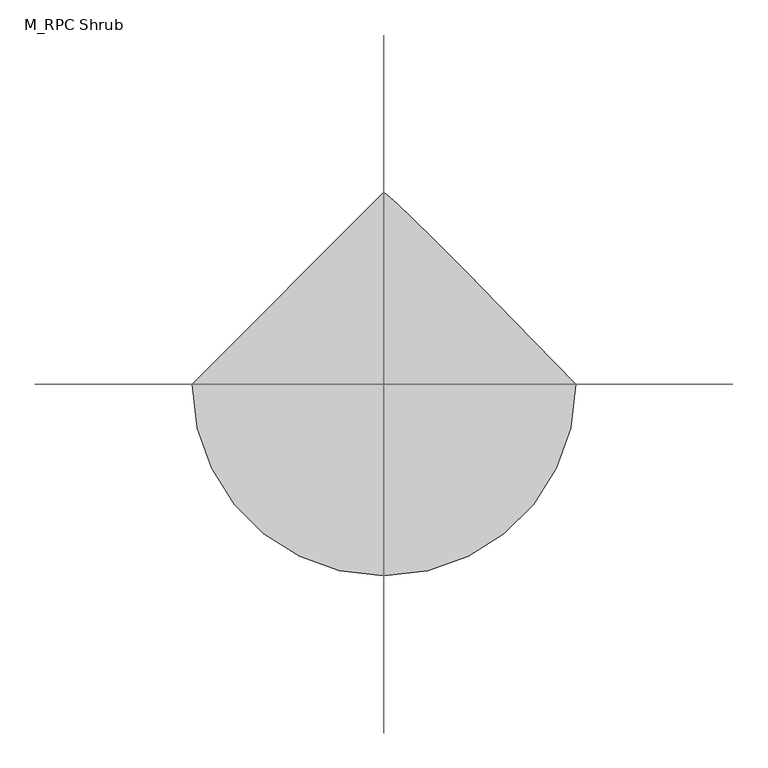
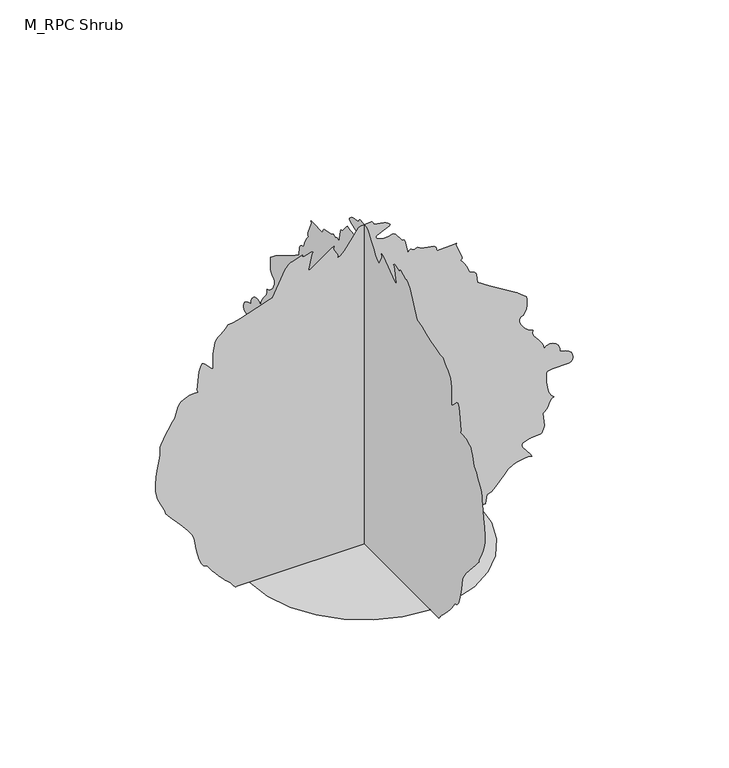
"""IFC4 building model written with IfcOpenShell, lengths in millimetres: geographic element geometry, M_RPC Shrub : Vibernum - 0.92 Meters."""

from ifc_helpers import new_model, si_unit, origin, place, context, project, spatial, triangles, source, transform, mapped, element, save


def m_rpc_shrub_8dd75232(model_context):
    return source(origin(), model_context, "Body", "Tessellation", [
        triangles([(-312.3019403, 0.0, 0.0), (-304.047466, -71.5591904, 0.0), (-280.533785, -137.2748422, 0.0), (-243.6445759, -195.2642804, 0.0), (-195.2642804, -243.6445759, 0.0), (-137.2748422, -280.533785, 0.0), (-71.5591904, -304.047466, 0.0), (1.37e-05, -312.3019403, 0.0), (71.5591904, -304.047466, 0.0), (137.2748422, -280.533785, 0.0), (195.2642804, -243.6445759, 0.0), (243.6445759, -195.2642804, 0.0), (280.533785, -137.2748422, 0.0), (304.047466, -71.5591904, 0.0), (312.3019403, 2.73e-05, 0.0), (210.8115327, 104.1055005, 0.0), (135.5708038, 180.7538289, 0.0), (82.2056472, 234.5209685, 0.0), (46.341203, 269.9844471, 0.0), (23.602184, 291.7169141, 0.0), (9.6134973, 304.2979231, 0.0), (-4.1e-05, 312.3019403, 0.0), (-354.9158363, 2.17e-05, 4.3761881), (-358.1767565, 2.14e-05, 8.534566), (-361.2817268, 2.12e-05, 12.3988753), (-364.2359797, 2.1e-05, 15.8927061), (-367.0419857, 2.08e-05, 18.9398516), (-369.7074117, 2.06e-05, 21.4638743), (-372.2322939, 2.05e-05, 23.3884638), (-378.1177631, 2.02e-05, 28.7068347), (-385.9096567, 1.97e-05, 36.5531626), (-394.8617629, 1.91e-05, 46.1891501), (-404.2381165, 1.85e-05, 56.876234), (-413.2898895, 1.79e-05, 67.8763802), (-421.2734502, 1.73e-05, 78.4512797), (-427.4502534, 1.67e-05, 87.8626239), (-436.9799043, 1.65e-05, 90.8633673), (-444.2223764, 1.6e-05, 99.7947807), (-449.6503881, 1.52e-05, 113.1020808), (-453.7290273, 1.42e-05, 129.2314832), (-456.9337008, 1.32e-05, 146.6279323), (-459.7294968, 1.22e-05, 163.737135), (-462.5891696, 1.12e-05, 179.0048078), (-468.7352697, 1.05e-05, 190.9709378), (-479.8672937, 9.6e-06, 206.3408391), (-493.9688676, 8.6e-06, 223.4354715), (-509.0261971, 7.6e-06, 240.5755953), (-523.0229808, 6.6e-06, 256.082207), (-533.9428811, 5.9e-06, 268.2773383), (-539.7695603, 5.5e-06, 275.4814407), (-541.2747737, 5.1e-06, 281.6198924), (-544.5919041, 4.7e-06, 289.5319094), (-548.9951237, 4.1e-06, 298.5044722), (-553.7612208, 3.6e-06, 307.832264), (-558.1644768, 3e-06, 316.8048268), (-561.4815708, 2.6e-06, 324.7142641), (-562.9867842, 2.2e-06, 330.8552773), (-567.5177939, 1.1e-06, 348.3710687), (-568.1004619, -1e-07, 369.3445341), (-565.9844573, -1.4e-06, 391.9765466), (-562.4143627, -2.8e-06, 414.4603486), (-558.6398111, -4e-06, 434.9916899), (-555.9053487, -5e-06, 451.7663564), (-555.4581376, -5.7e-06, 462.9801704), (-554.8294696, -6.3e-06, 472.6580681), (-551.5404625, -6.9e-06, 482.7883), (-546.3679948, -7.5e-06, 493.1791992), (-540.0966843, -8.1e-06, 503.6441854), (-533.5084236, -8.7e-06, 513.9839613), (-527.387867, -9.3e-06, 524.0119829), (-522.5144362, -9.9e-06, 533.5340034), (-517.8479696, -1.01e-05, 537.8503461), (-514.3085418, -1.06e-05, 545.0212383), (-511.4412023, -1.11e-05, 553.9068878), (-508.8013198, -1.17e-05, 563.3599082), (-505.9365237, -1.22e-05, 572.2430142), (-502.3945161, -1.26e-05, 579.4139065), (-497.7280858, -1.29e-05, 583.7328289), (-491.707196, -1.31e-05, 586.9451328), (-486.0159737, -1.33e-05, 589.7204721), (-480.370715, -1.34e-05, 591.9949336), (-474.4878256, -1.35e-05, 593.6994807), (-468.0810582, -1.35e-05, 594.7651497), (-460.8615861, -1.35e-05, 595.1254838), (-452.5509378, -1.35e-05, 594.7140627), (-454.8586095, -1.39e-05, 601.4453742), (-449.5864749, -1.7e-05, 652.1016209), (-445.5359227, -1.76e-05, 663.7626823), (-440.7468255, -1.81e-05, 672.2471209), (-437.1766946, -1.81e-05, 671.6951197), (-433.6142303, -1.8e-05, 669.1088676), (-417.0644411, -1.69e-05, 651.3937426), (-411.7642196, -1.67e-05, 648.3628956), (-411.5010089, -1.75e-05, 661.4268511), (-411.6236758, -1.81e-05, 670.3457834), (-411.8281328, -1.84e-05, 676.8215509), (-411.8102197, -1.88e-05, 682.5587734), (-411.2658852, -1.92e-05, 689.2594545), (-409.888462, -1.97e-05, 698.6281414), (-407.3712101, -2.05e-05, 712.3668377), (-405.7612066, -2.11e-05, 721.8709087), (-402.254989, -2.15e-05, 728.7811701), (-397.2435579, -2.18e-05, 734.1146381), (-391.1102114, -2.21e-05, 738.888402), (-384.2485299, -2.24e-05, 744.1247103), (-377.041884, -2.28e-05, 750.8407248), (-369.8786222, -2.34e-05, 760.056078), (-356.6894199, -2.34e-05, 760.8763767), (-337.3923783, -2.37e-05, 765.7038437), (-314.8319095, -2.42e-05, 772.9769463), (-291.8651246, -2.47e-05, 781.1368406), (-271.3388884, -2.51e-05, 788.6195234), (-256.1026636, -2.54e-05, 793.8635347), (-249.0097099, -2.55e-05, 795.3125742), (-214.9880765, -2.96e-05, 864.0289467), (-206.5153742, -3.02e-05, 874.8747236), (-198.5757789, -3.05e-05, 879.4338203), (-194.4166032, -3.05e-05, 879.2012764), (-169.7628755, -3.11e-05, 889.5334219), (-167.4802568, -3.11e-05, 888.8663841), (-169.1035589, -3.08e-05, 884.473411), (-162.8687651, -3.08e-05, 884.7749187), (-145.2576398, -3.11e-05, 890.2566336), (-141.9579048, -3.11e-05, 889.5691755), (-138.8076701, -3.09e-05, 886.8066261), (-141.6543078, -3.09e-05, 885.8252907), (-151.2105559, -2.84e-05, 843.1832714), (-151.3572493, -2.81e-05, 839.1173859), (-142.906784, -2.83e-05, 842.4907265), (-90.4708313, -3.06e-05, 880.7678232), (-82.020366, -3.08e-05, 884.1411638), (-83.7461328, -3.04e-05, 878.3323614), (-82.5360776, -3.01e-05, 872.9759296), (-73.0337507, -2.92e-05, 857.8138464), (-71.8234367, -2.89e-05, 852.457342), (-73.5492034, -2.85e-05, 846.6486122), (-63.9454201, -2.88e-05, 850.7834616), (-53.4106434, -2.94e-05, 861.4529411), (-42.6269584, -3.03e-05, 875.9301825), (-32.2761822, -3.12e-05, 891.4755999), (-23.0409855, -3.21e-05, 905.3650864), (-15.602804, -3.26e-05, 914.8640705), (-10.6438464, -3.27e-05, 917.2407423), (19.0264334, -3.29e-05, 920.0007483), (21.6640755, -3.29e-05, 918.7715355), (24.0025888, -3.27e-05, 915.4569849), (26.8484339, -3.23e-05, 909.3977617), (53.6932888, -3.21e-05, 905.3395065), (59.1330503, -3.19e-05, 902.9602913), (64.3586534, -3.17e-05, 899.3978634), (69.5170458, -3.14e-05, 894.3378525), (68.476934, -3.12e-05, 890.9466351), (63.7141433, -3.1e-05, 887.5732944), (34.9342185, -3.03e-05, 875.4190218), (32.1818815, -3.01e-05, 873.0040529), (32.3303599, -2.99e-05, 869.0122908), (35.7864966, -2.97e-05, 865.4217396), (41.7820881, -2.95e-05, 862.5365232), (49.5489423, -2.94e-05, 860.6632364), (58.3180791, -2.94e-05, 860.1163948), (67.3220762, -2.94e-05, 861.1973608), (75.7922169, -2.96e-05, 864.218034), (80.0229407, -2.96e-05, 864.2512442), (84.706512, -2.94e-05, 860.3745186), (99.6636841, -2.82e-05, 840.924107), (104.3475097, -2.8e-05, 837.0473814), (108.5782381, -2.8e-05, 837.0780481), (111.2337173, -2.77e-05, 832.0333706), (118.4610832, -2.55e-05, 796.4497868), (122.8172944, -2.58e-05, 801.0931807), (126.0518626, -2.59e-05, 802.5371332), (128.7277803, -2.59e-05, 801.9544653), (134.6612753, -2.58e-05, 799.3784597), (139.0463547, -2.58e-05, 799.7259676), (145.1290957, -2.59e-05, 802.7236771), (155.0420989, -2.55e-05, 796.4983303), (189.6435843, -2.52e-05, 789.5906851), (194.7493409, -2.48e-05, 784.3466738), (197.5241715, -2.42e-05, 774.4873192), (244.8328936, -2.43e-05, 775.7599886), (250.8604327, -2.44e-05, 776.9968317), (249.2693416, -2.41e-05, 771.5561028), (265.3001036, -2.18e-05, 733.5293541), (266.0080001, -2.14e-05, 726.8210426), (261.8424295, -2.12e-05, 723.9741234), (266.0591053, -2.1e-05, 720.0232744), (270.234886, -2.07e-05, 714.4291391), (274.257333, -2.03e-05, 707.7387045), (278.0191129, -1.98e-05, 700.503899), (281.4077868, -1.94e-05, 693.2690935), (284.3134598, -1.9e-05, 686.5812023), (286.6262365, -1.87e-05, 680.9922266), (293.9427957, -1.85e-05, 678.6513084), (299.3426841, -1.83e-05, 675.7763386), (303.1223589, -1.81e-05, 672.1142075), (305.5782592, -1.79e-05, 667.414567), (307.9625977, -1.65e-05, 644.5985178), (339.6157165, -1.52e-05, 623.0781744), (415.3650172, -1.24e-05, 576.2961462), (440.8030357, -1.13e-05, 556.8688073), (442.576583, -1.09e-05, 550.3086699), (442.6839166, -9.8e-06, 531.5483325), (440.8055792, -9.2e-06, 521.6711011), (437.4961518, -8.7e-06, 513.0077491), (432.650808, -8.3e-06, 506.7185254), (426.1647941, -8.1e-06, 503.9636427), (422.1781188, -7.8e-06, 498.3005073), (422.533366, -7.3e-06, 490.1891928), (426.3513379, -6.7e-06, 480.8102958), (432.7453517, -6.2e-06, 471.3393986), (440.8337025, -5.7e-06, 462.9545906), (449.7321419, -5.3e-06, 456.834034), (458.5564942, -5.1e-06, 454.1558181), (457.3502815, -4.7e-06, 446.192714), (460.7465858, -4.2e-06, 437.8002394), (467.069056, -3.7e-06, 429.0065901), (474.6386158, -3.1e-06, 419.8346935), (481.7788413, -2.5e-06, 410.312673), (486.8081855, -1.9e-06, 400.4635649), (488.0501882, -1.3e-06, 390.3103329), (495.6350813, -1.7e-06, 396.7784337), (504.4108538, -1.9e-06, 398.9378949), (513.4166631, -1.8e-06, 397.4173119), (521.6864345, -1.5e-06, 392.8454252), (528.2618689, -1.1e-06, 385.8534465), (532.179544, -5e-07, 377.0725508), (532.4734214, 0.0, 367.1314061), (546.6107852, 2e-07, 363.8347323), (556.6388068, 5e-07, 359.145302), (563.158031, 8e-07, 353.5384131), (566.7767055, 1.2e-06, 347.4894001), (568.1004619, 1.6e-06, 341.476177), (567.7299176, 1.9e-06, 335.9714985), (566.2732478, 2.1e-06, 331.4558221), (561.9262384, 2.4e-06, 327.0142691), (555.0594701, 2.5e-06, 325.3173886), (511.4182022, 2.5e-06, 325.4477222), (498.7170879, 2.7e-06, 322.0718382), (496.0746257, 3e-06, 317.2162479), (494.9374131, 3.7e-06, 306.5493482), (495.402501, 4.5e-06, 292.2791255), (497.5721724, 5.4e-06, 276.6186715), (501.5384274, 6.3e-06, 261.7785526), (507.4034037, 7e-06, 249.9677909), (515.2668772, 7.4e-06, 243.4002594), (509.294531, 7.7e-06, 239.3864964), (505.0855219, 8e-06, 233.7990286), (501.9447616, 8.4e-06, 227.2979356), (499.1745091, 8.8e-06, 220.5436059), (496.0848358, 9.1e-06, 214.1955922), (491.9806169, 9.5e-06, 208.9140286), (486.1667275, 9.7e-06, 205.3589949), (489.4889448, 1.19e-05, 168.9520057), (487.7639411, 1.24e-05, 160.1419693), (482.6553866, 1.3e-05, 150.3409051), (480.9687163, 1.31e-05, 148.301313), (450.9639344, 1.32e-05, 146.2540543), (429.6940118, 1.36e-05, 139.4731364), (428.2807986, 1.4e-05, 133.6410978), (430.2076796, 1.43e-05, 127.5542691), (451.9478133, 1.59e-05, 100.1517902), (456.0469454, 1.64e-05, 92.4117739), (449.7219317, 1.63e-05, 94.6872437), (435.3801473, 1.63e-05, 94.8479897), (418.8610248, 1.65e-05, 90.6992967), (417.1436877, 1.66e-05, 89.9019616), (403.775572, 1.67e-05, 86.4391824), (391.3376684, 1.73e-05, 77.4489881), (379.5693097, 1.81e-05, 65.0972075), (368.2072852, 1.89e-05, 51.5494334), (356.9832973, 1.96e-05, 38.9722533), (345.6366062, 2.02e-05, 29.5310031), (333.9040375, 2.04e-05, 25.3916891), (328.9564834, 2.19e-05, 4.03e-05), (-351.4939522, 2.19e-05, 4.03e-05), (-4.6e-06, -354.9158363, 4.3762136), (-4.6e-06, -358.1767565, 8.5345916), (-4.6e-06, -361.2817268, 12.3988753), (-4.6e-06, -364.2359797, 15.8927322), (-4.6e-06, -367.0419857, 18.9398766), (-4.6e-06, -369.7074117, 21.4638993), (-4.6e-06, -372.2322939, 23.3884638), (-4.6e-06, -378.1177631, 28.7068347), (-4.6e-06, -385.9096567, 36.5531626), (-4.6e-06, -394.8617629, 46.1891501), (-4.6e-06, -404.2381165, 56.876234), (-4.6e-06, -413.2898895, 67.8766345), (-4.6e-06, -421.2734502, 78.4512797), (-4.6e-06, -427.4502534, 87.8626239), (-4.6e-06, -436.9799043, 90.8633673), (-4.6e-06, -444.2223764, 99.7947807), (-4.6e-06, -449.6503881, 113.1023351), (-4.6e-06, -453.7290273, 129.2314832), (-4.6e-06, -456.9337008, 146.6279323), (-4.6e-06, -459.7294968, 163.737135), (-4.6e-06, -462.5891696, 179.0048078), (-4.6e-06, -468.7352697, 190.9709378), (-4.6e-06, -479.8672937, 206.3408391), (-4.6e-06, -493.9688676, 223.4354715), (-4.6e-06, -509.0261971, 240.5755953), (-4.6e-06, -523.0229808, 256.082207), (-4.6e-06, -533.9428811, 268.2773383), (-4.6e-06, -539.7695603, 275.4814407), (-4.6e-06, -541.2747737, 281.6198924), (-4.6e-06, -544.5919041, 289.5319094), (-4.6e-06, -548.9951237, 298.5044722), (-4.6e-06, -553.7612208, 307.832264), (-4.6e-06, -558.1644768, 316.8048268), (-4.6e-06, -561.4815708, 324.7142641), (-4.6e-06, -562.9867842, 330.8552773), (-4.6e-06, -567.5177939, 348.3710687), (-4.6e-06, -568.1004619, 369.3445341), (-4.6e-06, -565.9844573, 391.9765466), (-4.6e-06, -562.4143627, 414.4603486), (-4.6e-06, -558.6398111, 434.9916899), (-4.6e-06, -555.9053487, 451.7663564), (-4.6e-06, -555.4581376, 462.9801704), (-4.6e-06, -554.8294696, 472.6580681), (-4.6e-06, -551.5404625, 482.7883), (-4.6e-06, -546.3679948, 493.1791992), (-4.6e-06, -540.0966843, 503.6441854), (-4.6e-06, -533.5084236, 513.9839613), (-4.6e-06, -527.387867, 524.0119829), (-4.6e-06, -522.5144362, 533.5340034), (-4.6e-06, -517.8479696, 537.8503461), (-4.6e-06, -514.3085418, 545.0212383), (-4.6e-06, -511.4412023, 553.9068878), (-4.6e-06, -508.8013198, 563.3599082), (-4.6e-06, -505.9365237, 572.2430142), (-4.6e-06, -502.3945161, 579.4164863), (-4.6e-06, -497.7280858, 583.7328289), (-4.6e-06, -491.707196, 586.9451328), (-4.6e-06, -486.0159737, 589.7204721), (-4.6e-06, -480.370715, 591.9949336), (-4.6e-06, -474.4878256, 593.6994807), (-4.6e-06, -468.0810582, 594.7651497), (-4.6e-06, -460.8615861, 595.1254838), (-4.6e-06, -452.5509378, 594.7140627), (-4.6e-06, -454.8586095, 601.4453742), (-4.6e-06, -449.5864749, 652.1016209), (-4.6e-06, -445.5359227, 663.7626823), (-4.6e-06, -440.7468255, 672.2471209), (-4.6e-06, -437.1766946, 671.6951197), (-4.6e-06, -433.6142303, 669.1088676), (-4.6e-06, -417.0644411, 651.3937426), (-4.6e-06, -411.7642196, 648.3628956), (-4.6e-06, -411.5010089, 661.4268511), (-4.6e-06, -411.6236758, 670.3457834), (-4.6e-06, -411.8281328, 676.8215509), (-4.6e-06, -411.8102197, 682.5587734), (-4.6e-06, -411.2658852, 689.2594545), (-4.6e-06, -409.888462, 698.6281414), (-4.6e-06, -407.3712101, 712.3668377), (-4.6e-06, -405.7612066, 721.8709087), (-4.6e-06, -402.254989, 728.7811701), (-4.6e-06, -397.2435579, 734.1146381), (-4.6e-06, -391.1102114, 738.888402), (-4.6e-06, -384.2485299, 744.1247103), (-4.6e-06, -377.041884, 750.8407248), (-4.6e-06, -369.8786222, 760.056078), (-4.6e-06, -356.6894199, 760.8763767), (-4.6e-06, -337.3923783, 765.7038437), (-4.6e-06, -314.8319095, 772.9769463), (-4.6e-06, -291.8651246, 781.1368406), (-4.6e-06, -271.3388884, 788.6195234), (-4.6e-06, -256.1026636, 793.8635347), (-4.6e-06, -249.0097099, 795.3125742), (-4.6e-06, -214.9880765, 864.0289467), (-4.6e-06, -206.5153742, 874.8747236), (-4.6e-06, -198.5757789, 879.4338203), (-4.6e-06, -194.4166032, 879.2012764), (-4.6e-06, -169.7628755, 889.5334219), (-4.6e-06, -167.4800025, 888.8663841), (-4.6e-06, -169.1035589, 884.473411), (-4.6e-06, -162.8687651, 884.7749187), (-4.6e-06, -145.2576398, 890.2566336), (-4.6e-06, -141.9579048, 889.5691755), (-4.6e-06, -138.8076701, 886.8066261), (-4.6e-06, -141.6543078, 885.8252907), (-4.6e-06, -151.2105559, 843.1832714), (-4.6e-06, -151.3572493, 839.1199293), (-4.6e-06, -142.906784, 842.4907265), (-4.6e-06, -90.4708313, 880.7678232), (-4.6e-06, -82.020366, 884.1411638), (-4.6e-06, -83.7461328, 878.3323614), (-4.6e-06, -82.5360776, 872.9759296), (-4.6e-06, -73.0337507, 857.8138464), (-4.6e-06, -71.8234367, 852.457342), (-4.6e-06, -73.5492034, 846.6486122), (-4.6e-06, -63.9454201, 850.7834616), (-4.6e-06, -53.4106434, 861.4529411), (-4.6e-06, -42.6269584, 875.9301825), (-4.6e-06, -32.2761822, 891.4755999), (-4.6e-06, -23.0409855, 905.3650864), (-4.6e-06, -15.602804, 914.8640705), (-4.6e-06, -10.6438464, 917.2407423), (-4.6e-06, 19.0264334, 920.0007483), (-4.6e-06, 21.6640755, 918.7715355), (-4.6e-06, 24.0025888, 915.4569849), (-4.6e-06, 26.8484339, 909.3977617), (-4.6e-06, 53.6932888, 905.3395065), (-4.6e-06, 59.1330503, 902.9602913), (-4.6e-06, 64.3586534, 899.3978634), (-4.6e-06, 69.5170458, 894.3378525), (-4.6e-06, 68.476934, 890.9466351), (-4.6e-06, 63.7141433, 887.5758379), (-4.6e-06, 34.9342185, 875.4190218), (-4.6e-06, 32.1818815, 873.0040529), (-4.6e-06, 32.3303599, 869.0122908), (-4.6e-06, 35.7864966, 865.4217396), (-4.6e-06, 41.7820881, 862.5365232), (-4.6e-06, 49.5489423, 860.6658525), (-4.6e-06, 58.3180791, 860.1163948), (-4.6e-06, 67.3220762, 861.1973608), (-4.6e-06, 75.7922169, 864.218034), (-4.6e-06, 80.0229407, 864.2512442), (-4.6e-06, 84.706512, 860.3745186), (-4.6e-06, 99.6636841, 840.924107), (-4.6e-06, 104.3475097, 837.0473814), (-4.6e-06, 108.5782381, 837.0805916), (-4.6e-06, 111.2337173, 832.0333706), (-4.6e-06, 118.4610832, 796.4497868), (-4.6e-06, 122.8172944, 801.0931807), (-4.6e-06, 126.0518626, 802.5371332), (-4.6e-06, 128.7277803, 801.9544653), (-4.6e-06, 134.6612753, 799.3784597), (-4.6e-06, 139.0463547, 799.7259676), (-4.6e-06, 145.1290957, 802.7236771), (-4.6e-06, 155.0420989, 796.4983303), (-4.6e-06, 189.6435843, 789.5906851), (-4.6e-06, 194.7493409, 784.3466738), (-4.6e-06, 197.5241715, 774.4873192), (-4.6e-06, 244.8328936, 775.7599886), (-4.6e-06, 250.8604327, 776.9968317), (-4.6e-06, 249.2693416, 771.5561028), (-4.6e-06, 265.3001036, 733.5293541), (-4.6e-06, 266.0080001, 726.8210426), (-4.6e-06, 261.8424295, 723.9741234), (-4.6e-06, 266.0591053, 720.0232744), (-4.6e-06, 270.234886, 714.4291391), (-4.6e-06, 274.257333, 707.7387045), (-4.6e-06, 278.0191129, 700.503899), (-4.6e-06, 281.4077868, 693.2690935), (-4.6e-06, 284.3134598, 686.5812023), (-4.6e-06, 286.6262365, 680.9922266), (-4.6e-06, 293.9427957, 678.6513084), (-4.6e-06, 299.3426841, 675.7763386), (-4.6e-06, 303.1223589, 672.1142075), (-4.6e-06, 305.5782592, 667.414567), (-4.6e-06, 307.9625977, 644.5985178), (-4.6e-06, 339.6157165, 623.0781744), (-4.6e-06, 415.3650172, 576.2986897), (-4.6e-06, 440.8030357, 556.8688073), (-4.6e-06, 442.576583, 550.3086699), (-4.6e-06, 442.6839166, 531.5483325), (-4.6e-06, 440.8055792, 521.6711011), (-4.6e-06, 437.4961518, 513.0077491), (-4.6e-06, 432.650808, 506.7185254), (-4.6e-06, 426.1647941, 503.9636427), (-4.6e-06, 422.1781188, 498.3005073), (-4.6e-06, 422.533366, 490.1891928), (-4.6e-06, 426.3513379, 480.8102958), (-4.6e-06, 432.7453517, 471.3393986), (-4.6e-06, 440.8337025, 462.9545906), (-4.6e-06, 449.7321419, 456.834034), (-4.6e-06, 458.5564942, 454.1558181), (-4.6e-06, 457.3502815, 446.192714), (-4.6e-06, 460.7465858, 437.8002394), (-4.6e-06, 467.069056, 429.0065901), (-4.6e-06, 474.6386158, 419.8346935), (-4.6e-06, 481.7788413, 410.312673), (-4.6e-06, 486.8081855, 400.4635649), (-4.6e-06, 488.0501882, 390.3103329), (-4.6e-06, 495.6350813, 396.7784337), (-4.6e-06, 504.4108538, 398.9378949), (-4.6e-06, 513.4166631, 397.4173119), (-4.6e-06, 521.6864345, 392.8454252), (-4.6e-06, 528.2618689, 385.8534465), (-4.6e-06, 532.179544, 377.0725508), (-4.6e-06, 532.4734214, 367.1314061), (-4.6e-06, 546.6107852, 363.8347323), (-4.6e-06, 556.6388068, 359.145302), (-4.6e-06, 563.158031, 353.5384131), (-4.6e-06, 566.7767055, 347.4894001), (-4.6e-06, 568.1004619, 341.476177), (-4.6e-06, 567.7299176, 335.9714985), (-4.6e-06, 566.2732478, 331.4558221), (-4.6e-06, 561.9262384, 327.0142691), (-4.6e-06, 555.0594701, 325.3173886), (-4.6e-06, 511.4182022, 325.4477222), (-4.6e-06, 498.7170879, 322.0718382), (-4.6e-06, 496.0746257, 317.2162479), (-4.6e-06, 494.9374131, 306.5493482), (-4.6e-06, 495.402501, 292.2791255), (-4.6e-06, 497.5721724, 276.6186715), (-4.6e-06, 501.5384274, 261.7785526), (-4.6e-06, 507.4034037, 249.9680453), (-4.6e-06, 515.2668772, 243.4002594), (-4.6e-06, 509.294531, 239.3864964), (-4.6e-06, 505.0855219, 233.7990286), (-4.6e-06, 501.9447616, 227.2979356), (-4.6e-06, 499.1745091, 220.5436059), (-4.6e-06, 496.0848358, 214.1955922), (-4.6e-06, 491.9806169, 208.9140286), (-4.6e-06, 486.1667275, 205.3589949), (-4.6e-06, 489.4889448, 168.9520057), (-4.6e-06, 487.7639411, 160.1419693), (-4.6e-06, 482.6553866, 150.3409051), (-4.6e-06, 480.9687163, 148.3015674), (-4.6e-06, 450.9639344, 146.2540543), (-4.6e-06, 429.6940118, 139.4731364), (-4.6e-06, 428.2807986, 133.6413521), (-4.6e-06, 430.2076796, 127.5542691), (-4.6e-06, 451.9478133, 100.1517902), (-4.6e-06, 456.0469454, 92.4117739), (-4.6e-06, 449.7219317, 94.6872437), (-4.6e-06, 435.3801473, 94.8479897), (-4.6e-06, 418.8610248, 90.6992967), (-4.6e-06, 417.1436877, 89.9019616), (-4.6e-06, 403.775572, 86.4391824), (-4.6e-06, 391.3376684, 77.4489881), (-4.6e-06, 379.5693097, 65.0972075), (-4.6e-06, 368.2072852, 51.5494334), (-4.6e-06, 356.9832973, 38.9722533), (-4.6e-06, 345.6366062, 29.5310031), (-4.6e-06, 333.9040375, 25.3917141), (-4.6e-06, 328.9564834, 6.07e-05), (-4.6e-06, -351.4939522, 6.07e-05)], [[21, 22, 1], [20, 21, 1], [19, 20, 1], [18, 19, 1], [17, 18, 1], [17, 1, 2], [17, 2, 3], [17, 3, 4], [16, 17, 4], [16, 4, 5], [16, 5, 6], [16, 6, 7], [16, 7, 8], [16, 8, 9], [16, 9, 10], [16, 10, 11], [16, 11, 12], [15, 16, 12], [14, 15, 12], [13, 14, 12], [261, 262, 263], [130, 131, 132], [124, 125, 126], [180, 181, 182], [244, 245, 246], [119, 120, 121], [118, 119, 121], [212, 213, 214], [273, 274, 275], [123, 124, 126], [260, 261, 263], [88, 89, 90], [88, 90, 91], [260, 263, 264], [87, 88, 91], [87, 91, 92], [122, 123, 126], [166, 167, 168], [150, 151, 152], [150, 152, 153], [149, 150, 153], [148, 149, 153], [148, 153, 154], [147, 148, 154], [147, 154, 155], [87, 92, 93], [183, 184, 185], [122, 126, 127], [121, 122, 127], [174, 175, 176], [130, 132, 133], [129, 130, 133], [260, 264, 265], [129, 133, 134], [129, 134, 135], [129, 135, 136], [273, 275, 23], [86, 87, 93], [85, 86, 93], [273, 23, 24], [273, 24, 25], [273, 25, 26], [118, 121, 127], [118, 127, 128], [106, 107, 108], [273, 26, 27], [260, 265, 266], [260, 266, 267], [259, 260, 267], [244, 246, 247], [179, 180, 182], [273, 27, 28], [255, 256, 257], [162, 163, 164], [161, 162, 164], [117, 118, 128], [116, 117, 128], [115, 116, 128], [114, 115, 128], [273, 28, 29], [273, 29, 30], [273, 30, 31], [273, 31, 32], [273, 32, 33], [273, 33, 34], [273, 34, 35], [273, 35, 36], [161, 164, 165], [170, 171, 172], [169, 170, 172], [169, 172, 173], [254, 255, 257], [253, 254, 257], [252, 253, 257], [252, 257, 258], [243, 244, 247], [160, 161, 165], [36, 37, 38], [243, 247, 248], [36, 38, 39], [273, 36, 39], [273, 39, 40], [273, 40, 41], [273, 41, 42], [273, 42, 43], [273, 43, 44], [273, 44, 45], [273, 45, 46], [273, 46, 47], [272, 273, 47], [271, 272, 47], [270, 271, 47], [269, 270, 47], [268, 269, 47], [267, 268, 47], [259, 267, 47], [258, 259, 47], [252, 258, 47], [252, 47, 48], [252, 48, 49], [252, 49, 50], [252, 50, 51], [252, 51, 52], [252, 52, 53], [252, 53, 54], [252, 54, 55], [252, 55, 56], [252, 56, 57], [252, 57, 58], [252, 58, 59], [252, 59, 60], [252, 60, 61], [252, 61, 62], [252, 62, 63], [252, 63, 64], [252, 64, 65], [252, 65, 66], [252, 66, 67], [252, 67, 68], [252, 68, 69], [252, 69, 70], [252, 70, 71], [252, 71, 72], [252, 72, 73], [252, 73, 74], [252, 74, 75], [252, 75, 76], [252, 76, 77], [252, 77, 78], [252, 78, 79], [252, 79, 80], [252, 80, 81], [252, 81, 82], [252, 82, 83], [252, 83, 84], [252, 84, 85], [252, 85, 93], [252, 93, 94], [252, 94, 95], [252, 95, 96], [252, 96, 97], [252, 97, 98], [252, 98, 99], [252, 99, 100], [252, 100, 101], [252, 101, 102], [252, 102, 103], [252, 103, 104], [252, 104, 105], [252, 105, 106], [252, 106, 108], [252, 108, 109], [252, 109, 110], [252, 110, 111], [252, 111, 112], [252, 112, 113], [252, 113, 114], [252, 114, 128], [252, 128, 129], [252, 129, 136], [252, 136, 137], [252, 137, 138], [251, 252, 138], [250, 251, 138], [249, 250, 138], [248, 249, 138], [243, 248, 138], [242, 243, 138], [241, 242, 138], [240, 241, 138], [239, 240, 138], [238, 239, 138], [238, 138, 139], [238, 139, 140], [238, 140, 141], [238, 141, 142], [238, 142, 143], [237, 238, 143], [234, 235, 236], [233, 234, 236], [232, 233, 236], [231, 232, 236], [230, 231, 236], [229, 230, 236], [228, 229, 236], [227, 228, 236], [227, 236, 237], [179, 182, 183], [179, 183, 185], [199, 200, 201], [199, 201, 202], [199, 202, 203], [199, 203, 204], [199, 204, 205], [199, 205, 206], [199, 206, 207], [198, 199, 207], [198, 207, 208], [144, 145, 146], [144, 146, 147], [144, 147, 155], [143, 144, 155], [143, 155, 156], [237, 143, 156], [237, 156, 157], [237, 157, 158], [237, 158, 159], [237, 159, 160], [177, 178, 179], [226, 227, 237], [225, 226, 237], [224, 225, 237], [223, 224, 237], [222, 223, 237], [221, 222, 237], [220, 221, 237], [220, 237, 160], [219, 220, 160], [218, 219, 160], [166, 168, 169], [165, 166, 169], [160, 165, 169], [218, 160, 169], [217, 218, 169], [216, 217, 169], [215, 216, 169], [215, 169, 173], [215, 173, 174], [215, 174, 176], [211, 212, 214], [211, 214, 215], [194, 195, 196], [193, 194, 196], [192, 193, 196], [192, 196, 197], [197, 198, 208], [176, 177, 179], [197, 208, 209], [176, 179, 185], [185, 186, 187], [176, 185, 187], [176, 187, 188], [176, 188, 189], [176, 189, 190], [176, 190, 191], [176, 191, 192], [176, 192, 197], [176, 197, 209], [176, 209, 210], [215, 176, 210], [211, 215, 210], [514, 515, 516], [383, 384, 385], [377, 378, 379], [433, 434, 435], [497, 498, 499], [372, 373, 374], [371, 372, 374], [465, 466, 467], [526, 527, 528], [376, 377, 379], [513, 514, 516], [341, 342, 343], [341, 343, 344], [513, 516, 517], [340, 341, 344], [340, 344, 345], [375, 376, 379], [419, 420, 421], [403, 404, 405], [403, 405, 406], [402, 403, 406], [401, 402, 406], [401, 406, 407], [400, 401, 407], [400, 407, 408], [340, 345, 346], [436, 437, 438], [375, 379, 380], [374, 375, 380], [427, 428, 429], [383, 385, 386], [382, 383, 386], [513, 517, 518], [382, 386, 387], [382, 387, 388], [382, 388, 389], [526, 528, 276], [339, 340, 346], [338, 339, 346], [526, 276, 277], [526, 277, 278], [526, 278, 279], [371, 374, 380], [371, 380, 381], [359, 360, 361], [526, 279, 280], [513, 518, 519], [513, 519, 520], [512, 513, 520], [497, 499, 500], [432, 433, 435], [526, 280, 281], [508, 509, 510], [415, 416, 417], [414, 415, 417], [370, 371, 381], [369, 370, 381], [368, 369, 381], [367, 368, 381], [526, 281, 282], [526, 282, 283], [526, 283, 284], [526, 284, 285], [526, 285, 286], [526, 286, 287], [526, 287, 288], [526, 288, 289], [414, 417, 418], [423, 424, 425], [422, 423, 425], [422, 425, 426], [507, 508, 510], [506, 507, 510], [505, 506, 510], [505, 510, 511], [496, 497, 500], [413, 414, 418], [289, 290, 291], [496, 500, 501], [289, 291, 292], [526, 289, 292], [526, 292, 293], [526, 293, 294], [526, 294, 295], [526, 295, 296], [526, 296, 297], [526, 297, 298], [526, 298, 299], [526, 299, 300], [525, 526, 300], [524, 525, 300], [523, 524, 300], [522, 523, 300], [521, 522, 300], [520, 521, 300], [512, 520, 300], [511, 512, 300], [505, 511, 300], [505, 300, 301], [505, 301, 302], [505, 302, 303], [505, 303, 304], [505, 304, 305], [505, 305, 306], [505, 306, 307], [505, 307, 308], [505, 308, 309], [505, 309, 310], [505, 310, 311], [505, 311, 312], [505, 312, 313], [505, 313, 314], [505, 314, 315], [505, 315, 316], [505, 316, 317], [505, 317, 318], [505, 318, 319], [505, 319, 320], [505, 320, 321], [505, 321, 322], [505, 322, 323], [505, 323, 324], [505, 324, 325], [505, 325, 326], [505, 326, 327], [505, 327, 328], [505, 328, 329], [505, 329, 330], [505, 330, 331], [505, 331, 332], [505, 332, 333], [505, 333, 334], [505, 334, 335], [505, 335, 336], [505, 336, 337], [505, 337, 338], [505, 338, 346], [505, 346, 347], [505, 347, 348], [505, 348, 349], [505, 349, 350], [505, 350, 351], [505, 351, 352], [505, 352, 353], [505, 353, 354], [505, 354, 355], [505, 355, 356], [505, 356, 357], [505, 357, 358], [505, 358, 359], [505, 359, 361], [505, 361, 362], [505, 362, 363], [505, 363, 364], [505, 364, 365], [505, 365, 366], [505, 366, 367], [505, 367, 381], [505, 381, 382], [505, 382, 389], [505, 389, 390], [505, 390, 391], [504, 505, 391], [503, 504, 391], [502, 503, 391], [501, 502, 391], [496, 501, 391], [495, 496, 391], [494, 495, 391], [493, 494, 391], [492, 493, 391], [491, 492, 391], [491, 391, 392], [491, 392, 393], [491, 393, 394], [491, 394, 395], [491, 395, 396], [490, 491, 396], [487, 488, 489], [486, 487, 489], [485, 486, 489], [484, 485, 489], [483, 484, 489], [482, 483, 489], [481, 482, 489], [480, 481, 489], [480, 489, 490], [432, 435, 436], [432, 436, 438], [452, 453, 454], [452, 454, 455], [452, 455, 456], [452, 456, 457], [452, 457, 458], [452, 458, 459], [452, 459, 460], [451, 452, 460], [451, 460, 461], [397, 398, 399], [397, 399, 400], [397, 400, 408], [396, 397, 408], [396, 408, 409], [490, 396, 409], [490, 409, 410], [490, 410, 411], [490, 411, 412], [490, 412, 413], [430, 431, 432], [479, 480, 490], [478, 479, 490], [477, 478, 490], [476, 477, 490], [475, 476, 490], [474, 475, 490], [473, 474, 490], [473, 490, 413], [472, 473, 413], [471, 472, 413], [419, 421, 422], [418, 419, 422], [413, 418, 422], [471, 413, 422], [470, 471, 422], [469, 470, 422], [468, 469, 422], [468, 422, 426], [468, 426, 427], [468, 427, 429], [464, 465, 467], [464, 467, 468], [447, 448, 449], [446, 447, 449], [445, 446, 449], [445, 449, 450], [450, 451, 461], [429, 430, 432], [450, 461, 462], [429, 432, 438], [438, 439, 440], [429, 438, 440], [429, 440, 441], [429, 441, 442], [429, 442, 443], [429, 443, 444], [429, 444, 445], [429, 445, 450], [429, 450, 462], [429, 462, 463], [468, 429, 463], [464, 468, 463]], closed=False),
    ])


if __name__ == "__main__":
    model = new_model("IFC4")
    model_context = context("Model", 3, world=origin())
    ifc_project = project(units=[si_unit("LENGTHUNIT", "METRE", prefix="MILLI")], contexts=[model_context])
    site = spatial("IfcSite", under=ifc_project)
    building = spatial("IfcBuilding", under=site)
    placement = place(None, origin())
    m_rpc_shrub_shape = m_rpc_shrub_8dd75232(model_context)
    element("IfcGeographicElement", 1, ObjectType="M_RPC Shrub : Vibernum - 0.92 Meters", at=placement, inside=building, context=model_context, shape_type="MappedRepresentation", body=[
        mapped(m_rpc_shrub_shape, transform((0.0, 0.0, 0.0), x_axis=(1.0, 0.0, 0.0), y_axis=(0.0, 1.0, 0.0), z_axis=(0.0, 0.0, 1.0))),
    ])
    save(model, "model.ifc")

# Revit data of these elements
# Type "M_RPC Shrub : Vibernum - 0.92 Meters"
#   Type Comments = "Vibernum"
#   built-in parameter 1005198 = "{2, 15},{39, RPC-16-FU5P-8RFX-7Q0N-4000-ST1L-LVER-AU},{1, 0},{1, 0},{2, 35},{1, 8},{5, Color},{1, 0},{1, 0},{3, 0.8},{3, 0.8},{3, 0.8},{1, 8},{7, BBoxMin},{1, 0},{1, 0},{1, 0},{1, 0},{1, 0},{1, 8},{7, BBoxMax},{1, 0},{1, 0},{1, 0},{1, 0},{1, 0},{2, 11},{9, RPCTypeId},{1, 0},{1, 0},{39, RPC-16-FU5P-8RFX-7Q0N-4000-ST1L-LVER-AU},{1, 6},{14, RPCPlantHeight},{1, 0},{1, 0},{7, 3.01837},{2, 11},{7, keyword},{1, 0},{1, 0},{22, :Geometry:RPC:Vibernum},{2, 11},{8, category},{1, 0},{1, 0},{17, :Shrubs & Grasses},{2, 11},{12, LocalizedUID},{1, 0},{1, 0},{8, Vibernum},{2, 14},{6, Height},{1, 0},{1, 0},{7, 3.01837},{1, 2},{16, Cast Reflections},{1, 0},{1, 0},{1, 0},{1, 2},{12, Cast Shadows},{1, 0},{1, 0},{1, 1},{1, 2},{9, Lock View},{1, 0},{1, 0},{1, 0},{1, 4},{5, ViewC},{1, 0},{1, 0},{1, 0},{2, 11},{20, AdvancedUIDefinition},{1, 0},{1, 0},{0, },{2, 11},{10, AssetLibID},{1, 0},{1, 0},{36, 4D3F6E72-3F99-4203-98E9-AF80B3C7A7A4},{2, 11},{10, BaseSchema},{1, 0},{1, 0},{9, RPCSchema},{2, 11},{12, ExchangeGUID},{1, 0},{1, 0},{0, },{1, 2},{6, Hidden},{1, 0},{1, 0},{1, 0},{1, 4},{11, RPCCategory},{1, 0},{1, 0},{1, 0},{2, 11},{8, RPCImage},{1, 0},{1, 0},{0, },{1, 4},{13, SchemaVersion},{1, 0},{1, 0},{1, 4},{2, 11},{12, UIDefinition},{1, 0},{1, 0},{0, },{2, 11},{6, UIName},{1, 0},{1, 0},{39, RPC-16-FU5P-8RFX-7Q0N-4000-ST1L-LVER-AU},{2, 11},{11, VersionGUID},{1, 0},{1, 0},{9, RPCSchema},{2, 11},{9, assettype},{1, 0},{1, 0},{11, RPCGeometry},{2, 11},{11, description},{1, 0},{1, 0},{0, },{2, 11},{9, localname},{1, 0},{1, 0},{3, RPC},{2, 11},{9, localtype},{1, 0},{1, 0},{3, RPC},{1, 4},{8, revision},{1, 0},{1, 0},{1, 1},{2, 11},{9, thumbnail},{1, 0},{1, 0},{0, },{1, 4},{7, version},{1, 0},{1, 0},{1, 1},{1, 2},{20, RPC_Cast Reflections},{1, 0},{1, 0},{1, 1},{1, 2},{16, RPC_Cast Shadows},{1, 0},{1, 0},{1, 1},{1, 2},{13, RPC_Lock View},{1, 0},{1, 0},{1, 0},{1, 4},{9, RPC_ViewC},{1, 0},{1, 0},{1, 0},{21, assetlibrary_base.fbx},{1, 5},"
#   built-in parameter 1005195 = "RPC-16-FU5P-8RFX-7Q0N-4000-ST1L-LVER-AU"
#   Height = 0.92 m
#   Description = (empty or 0)
